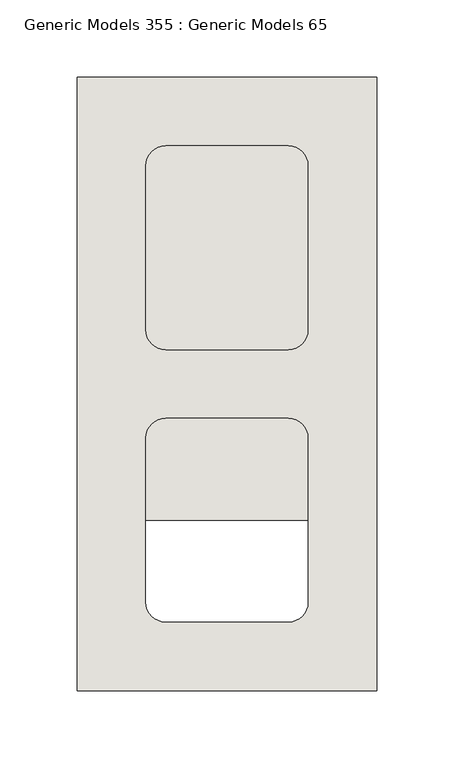
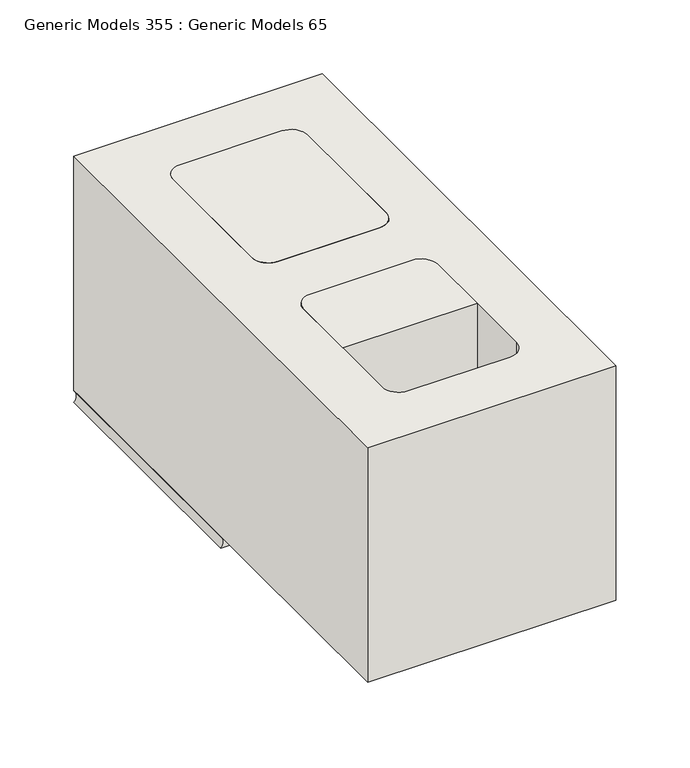
"""IFC4 building model written with IfcOpenShell, lengths in millimetres: wall geometry, Generic Models 355 : Generic Models 65."""

from ifc_helpers import new_model, si_unit, point, frame, frame_2d, origin, place, context, project, spatial, polyline, circle_curve, trimmed, segment, composite_curve, outline, extrude, source, transform, mapped, element, save
from ifc_brep_helpers import plane_surface, revolved_surface, advanced_brep


def generic_models_355_generic_models_65_aa9cf15c(model_context):
    return source(origin(), model_context, "Body", "SolidModel", [
        advanced_brep(
        [(430198.2125, 503.2375, 1838.325), (430004.5375, 503.2375, 1838.325), (430004.5375, 503.2375, 1828.8), (430198.2125, 503.2375, 1828.8), (430198.2125, 701.675, 1838.325), (430198.2125, 701.675, 1828.8), (430004.5375, 701.675, 1828.8), (430004.5375, 701.675, 1838.325), (430153.7625, 538.1625, 1838.325), (430141.0625, 525.4625, 1838.325), (430061.6875, 525.4625, 1838.325), (430048.9875, 538.1625, 1838.325), (430048.9875, 644.525, 1838.325), (430061.6875, 657.225, 1838.325), (430141.0625, 657.225, 1838.325), (430153.7625, 644.525, 1838.325), (430141.0625, 525.4625, 1828.8), (430153.7625, 538.1625, 1828.8), (430061.6875, 525.4625, 1828.8), (430048.9875, 538.1625, 1828.8), (430048.9875, 644.525, 1828.8), (430061.6875, 657.225, 1828.8), (430141.0625, 657.225, 1828.8), (430153.7625, 644.525, 1828.8)],
        [
            (0, 1),
            (1, 2, circle_curve(frame((429999.6545028, 503.2375, 1833.5625), z_axis=(0.0, 1.0, 0.0), x_axis=(1.0, 0.0, 0.0)), 6.8209287)),
            (2, 3),
            (3, 0, circle_curve(frame((430203.0954972, 503.2375, 1833.5625), z_axis=(0.0, 1.0, 0.0), x_axis=(-1.0, 0.0, 0.0)), 6.8209287)),
            (4, 5, circle_curve(frame((430203.0954972, 701.675, 1833.5625), z_axis=(0.0, -1.0, 0.0), x_axis=(-1.0, 0.0, 0.0)), 6.8209287)),
            (5, 6),
            (6, 7, circle_curve(frame((429999.6545028, 701.675, 1833.5625), z_axis=(0.0, -1.0, 0.0), x_axis=(1.0, 0.0, 0.0)), 6.8209287)),
            (7, 4),
            (0, 4),
            (7, 1),
            (8, 9, circle_curve(frame((430141.0625, 538.1625, 1838.325), z_axis=(0.0, 0.0, -1.0), x_axis=(-1.0, 0.0, 0.0)), 12.7)),
            (9, 10),
            (10, 11, circle_curve(frame((430061.6875, 538.1625, 1838.325), z_axis=(0.0, 0.0, -1.0), x_axis=(-1.0, 0.0, 0.0)), 12.7)),
            (11, 12),
            (12, 13, circle_curve(frame((430061.6875, 644.525, 1838.325), z_axis=(0.0, 0.0, -1.0), x_axis=(-1.0, 0.0, 0.0)), 12.7)),
            (13, 14),
            (14, 15, circle_curve(frame((430141.0625, 644.525, 1838.325), z_axis=(0.0, 0.0, -1.0), x_axis=(-1.0, 0.0, 0.0)), 12.7)),
            (15, 8),
            (16, 9),
            (8, 17),
            (17, 16, circle_curve(frame((430141.0625, 538.1625, 1828.8), z_axis=(0.0, 0.0, -1.0), x_axis=(-1.0, 0.0, 0.0)), 12.7)),
            (16, 18),
            (18, 10),
            (18, 19, circle_curve(frame((430061.6875, 538.1625, 1828.8), z_axis=(0.0, 0.0, -1.0), x_axis=(-1.0, 0.0, 0.0)), 12.7)),
            (19, 11),
            (19, 20),
            (20, 12),
            (20, 21, circle_curve(frame((430061.6875, 644.525, 1828.8), z_axis=(0.0, 0.0, -1.0), x_axis=(-1.0, 0.0, 0.0)), 12.7)),
            (21, 13),
            (21, 22),
            (22, 14),
            (22, 23, circle_curve(frame((430141.0625, 644.525, 1828.8), z_axis=(0.0, 0.0, -1.0), x_axis=(-1.0, 0.0, 0.0)), 12.7)),
            (23, 15),
            (23, 17),
            (6, 2),
            (5, 3),
        ],
        [
            plane_surface(frame((430101.375, 503.2375, 1838.721875), z_axis=(0.0, -1.0, 0.0), x_axis=(0.0, 0.0, 1.0))),
            plane_surface(frame((430101.375, 701.675, 1838.721875), z_axis=(0.0, 1.0, 0.0), x_axis=(0.0, 0.0, 1.0))),
            plane_surface(frame((430198.2125, 503.2375, 1838.325), z_axis=(0.0, 0.0, 1.0), x_axis=(0.0, 1.0, 0.0))),
            revolved_surface(polyline([(430128.3625, 538.1625, 1838.325), (430128.3625, 538.1625, 1828.8)]), (430141.0625, 538.1625, 2022.475), (0.0, 0.0, 1.0)),
            plane_surface(frame((430061.6875, 525.4625, 2022.475), z_axis=(0.0, 1.0, 0.0), x_axis=(0.0, 0.0, -1.0))),
            revolved_surface(polyline([(430048.9875, 538.1625, 1838.325), (430048.9875, 538.1625, 1828.8)]), (430061.6875, 538.1625, 2022.475), (0.0, 0.0, 1.0)),
            plane_surface(frame((430048.9875, 644.525, 2022.475), z_axis=(1.0, 0.0, 0.0), x_axis=(0.0, 0.0, -1.0))),
            revolved_surface(polyline([(430048.9875, 644.525, 1838.325), (430048.9875, 644.525, 1828.8)]), (430061.6875, 644.525, 2022.475), (0.0, 0.0, 1.0)),
            plane_surface(frame((430141.0625, 657.225, 2022.475), z_axis=(0.0, -1.0, 0.0), x_axis=(0.0, 0.0, -1.0))),
            revolved_surface(polyline([(430128.3625, 644.525, 1838.325), (430128.3625, 644.525, 1828.8)]), (430141.0625, 644.525, 2022.475), (0.0, 0.0, 1.0)),
            plane_surface(frame((430153.7625, 538.1625, 2022.475), z_axis=(-1.0, 0.0, 0.0), x_axis=(0.0, 0.0, -1.0))),
            revolved_surface(polyline([(430006.4754315, 701.675, 1833.5625), (430006.4754315, 503.2375, 1833.5625)]), (429999.6545028, 503.2375, 1833.5625), (0.0, 1.0, 0.0)),
            plane_surface(frame((430004.5375, 503.2375, 1828.8), z_axis=(0.0, 0.0, -1.0), x_axis=(0.0, 1.0, 0.0))),
            revolved_surface(polyline([(430196.2745685, 701.675, 1833.5625), (430196.2745685, 503.2375, 1833.5625)]), (430203.0954972, 503.2375, 1833.5625), (0.0, 1.0, 0.0)),
        ],
        [
            (0, [[1, 2, 3, 4]]),
            (1, [[5, 6, 7, 8]]),
            (2, [[-1, 9, -8, 10], [11, 12, 13, 14, 15, 16, 17, 18]]),
            (3, [[19, -11, 20, 21]]),
            (4, [[-19, 22, 23, -12]]),
            (5, [[-23, 24, 25, -13]]),
            (6, [[-25, 26, 27, -14]]),
            (7, [[-27, 28, 29, -15]]),
            (8, [[-29, 30, 31, -16]]),
            (9, [[-31, 32, 33, -17]]),
            (10, [[-33, 34, -20, -18]]),
            (11, [[-2, -10, -7, 35]]),
            (12, [[-3, -35, -6, 36], [-21, -34, -32, -30, -28, -26, -24, -22]]),
            (13, [[-4, -36, -5, -9]]),
        ],
    ),
        extrude(outline(composite_curve([segment(trimmed(circle_curve(frame_2d((430141.0625, 538.1625)), 12.7), [point((430153.7625, 538.1625))], [point((430141.0625, 525.4625))], False, "CARTESIAN"), True, "CONTINUOUS"), segment(polyline([(430141.0625, 525.4625), (430061.6875, 525.4625)]), True, "CONTINUOUS"), segment(trimmed(circle_curve(frame_2d((430061.6875, 538.1625)), 12.7), [point((430061.6875, 525.4625))], [point((430048.9875, 538.1625))], False, "CARTESIAN"), True, "CONTINUOUS"), segment(polyline([(430048.9875, 538.1625), (430048.9875, 644.525)]), True, "CONTINUOUS"), segment(trimmed(circle_curve(frame_2d((430061.6875, 644.525)), 12.7), [point((430048.9875, 644.525))], [point((430061.6875, 657.225))], False, "CARTESIAN"), True, "CONTINUOUS"), segment(polyline([(430061.6875, 657.225), (430141.0625, 657.225)]), True, "CONTINUOUS"), segment(trimmed(circle_curve(frame_2d((430141.0625, 644.525)), 12.7), [point((430141.0625, 657.225))], [point((430153.7625, 644.525))], False, "CARTESIAN"), True, "CONTINUOUS"), segment(polyline([(430153.7625, 644.525), (430153.7625, 538.1625)]), True, "CONTINUOUS")], self_intersect=False)), frame((0.0, 0.0, 1828.8), z_axis=(0.0, 0.0, 1.0), x_axis=(1.0, 0.0, 0.0)), (0.0, 0.0, 1.0), 203.2),
        extrude(outline(composite_curve([segment(trimmed(circle_curve(frame_2d((430061.6875, 468.3125)), 12.7), [point((430048.9875, 468.3125))], [point((430061.6875, 481.0125))], False, "CARTESIAN"), True, "CONTINUOUS"), segment(polyline([(430061.6875, 481.0125), (430141.0625, 481.0125)]), True, "CONTINUOUS"), segment(trimmed(circle_curve(frame_2d((430141.0625, 468.3125)), 12.7), [point((430141.0625, 481.0125))], [point((430153.7625, 468.3125))], False, "CARTESIAN"), True, "CONTINUOUS"), segment(polyline([(430153.7625, 468.3125), (430153.7625, 415.13125), (430048.9875, 415.13125), (430048.9875, 468.3125)]), True, "CONTINUOUS")], self_intersect=False)), frame((0.0, 0.0, 1828.8), z_axis=(0.0, 0.0, 1.0), x_axis=(1.0, 0.0, 0.0)), (0.0, 0.0, 1.0), 203.2),
        extrude(outline(polyline([(430198.2125, 304.8), (430004.5375, 304.8), (430004.5375, 701.675), (430198.2125, 701.675), (430198.2125, 304.8)]), holes=[composite_curve([segment(polyline([(430153.7625, 538.1625), (430153.7625, 644.525)]), True, "CONTINUOUS"), segment(trimmed(circle_curve(frame_2d((430141.0625, 644.525)), 12.7), [point((430153.7625, 644.525))], [point((430141.0625, 657.225))], True, "CARTESIAN"), True, "CONTINUOUS"), segment(polyline([(430141.0625, 657.225), (430061.6875, 657.225)]), True, "CONTINUOUS"), segment(trimmed(circle_curve(frame_2d((430061.6875, 644.525)), 12.7), [point((430061.6875, 657.225))], [point((430048.9875, 644.525))], True, "CARTESIAN"), True, "CONTINUOUS"), segment(polyline([(430048.9875, 644.525), (430048.9875, 538.1625)]), True, "CONTINUOUS"), segment(trimmed(circle_curve(frame_2d((430061.6875, 538.1625)), 12.7), [point((430048.9875, 538.1625))], [point((430061.6875, 525.4625))], True, "CARTESIAN"), True, "CONTINUOUS"), segment(polyline([(430061.6875, 525.4625), (430141.0625, 525.4625)]), True, "CONTINUOUS"), segment(trimmed(circle_curve(frame_2d((430141.0625, 538.1625)), 12.7), [point((430141.0625, 525.4625))], [point((430153.7625, 538.1625))], True, "CARTESIAN"), True, "CONTINUOUS")], self_intersect=False), composite_curve([segment(polyline([(430048.9875, 468.3125), (430048.9875, 361.95)]), True, "CONTINUOUS"), segment(trimmed(circle_curve(frame_2d((430061.6875, 361.95)), 12.7), [point((430048.9875, 361.95))], [point((430061.6875, 349.25))], True, "CARTESIAN"), True, "CONTINUOUS"), segment(polyline([(430061.6875, 349.25), (430141.0625, 349.25)]), True, "CONTINUOUS"), segment(trimmed(circle_curve(frame_2d((430141.0625, 361.95)), 12.7), [point((430141.0625, 349.25))], [point((430153.7625, 361.95))], True, "CARTESIAN"), True, "CONTINUOUS"), segment(polyline([(430153.7625, 361.95), (430153.7625, 468.3125)]), True, "CONTINUOUS"), segment(trimmed(circle_curve(frame_2d((430141.0625, 468.3125)), 12.7), [point((430153.7625, 468.3125))], [point((430141.0625, 481.0125))], True, "CARTESIAN"), True, "CONTINUOUS"), segment(polyline([(430141.0625, 481.0125), (430061.6875, 481.0125)]), True, "CONTINUOUS"), segment(trimmed(circle_curve(frame_2d((430061.6875, 468.3125)), 12.7), [point((430061.6875, 481.0125))], [point((430048.9875, 468.3125))], True, "CARTESIAN"), True, "CONTINUOUS")], self_intersect=False)]), frame((0.0, 0.0, 1838.325), z_axis=(0.0, 0.0, 1.0), x_axis=(1.0, 0.0, 0.0)), (0.0, 0.0, 1.0), 193.675),
    ])


if __name__ == "__main__":
    model = new_model("IFC4")
    model_context = context("Model", 3, world=origin())
    ifc_project = project(units=[si_unit("LENGTHUNIT", "METRE", prefix="MILLI")], contexts=[model_context])
    site = spatial("IfcSite", under=ifc_project)
    building = spatial("IfcBuilding", under=site)
    placement = place(None, origin())
    generic_models_355_generic_models_65_shape = generic_models_355_generic_models_65_aa9cf15c(model_context)
    element("IfcWall", 1, ObjectType="Generic Models 355 : Generic Models 65", at=placement, inside=building, context=model_context, shape_type="MappedRepresentation", body=[
        mapped(generic_models_355_generic_models_65_shape, transform((0.0, 0.0, 0.0), x_axis=(1.0, 0.0, 0.0), y_axis=(0.0, 1.0, 0.0), z_axis=(0.0, 0.0, 1.0))),
    ])
    save(model, "model.ifc")

# Revit data of these elements
# Element 1 (IfcWall, "Generic Models 355 : Generic Models 65")
#   Materials on its faces: "CMU (SEE 'WALL TAG' FOR SIZE)", "FILL CORE IF APPLICABLE - SEE STRUCTURAL DWGS FOR DETAILS", "MORTAR JOINT"
# Materials
#   "CMU (SEE 'WALL TAG' FOR SIZE)": class "Masonry", colour RGB 203 203 199, transparency 0, Description = "Concrete masonry units", Cost = 0
#   "FILL CORE IF APPLICABLE - SEE STRUCTURAL DWGS FOR DETAILS": class "Generic", colour RGB 170 170 170, transparency 0, Cost = 0
#   "MORTAR JOINT": class "Generic", colour RGB 120 120 120, transparency 0, Cost = 0
